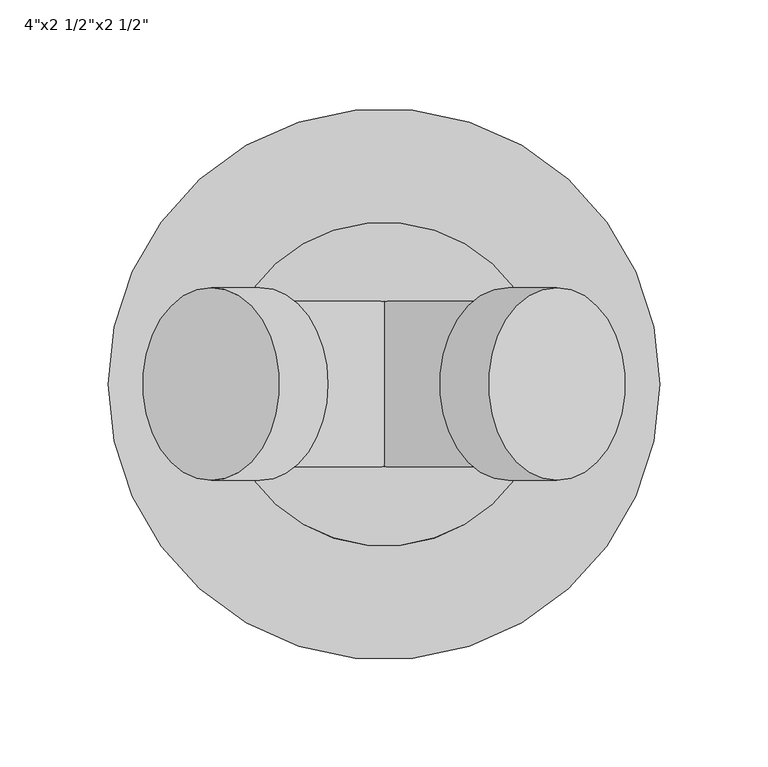
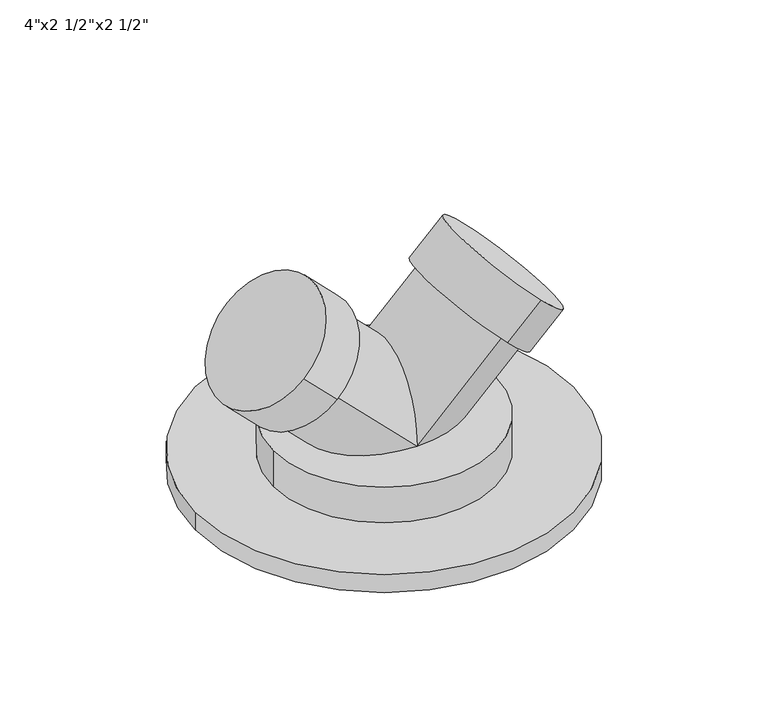
"""IFC4 building model written with IfcOpenShell, lengths in millimetres: proxy geometry."""

from ifc_helpers import new_model, si_unit, frame, origin, place, context, project, spatial, circle_curve, ellipse_curve, source, transform, mapped, element, save
from ifc_brep_helpers import plane_surface, cylinder_surface, advanced_brep


def proxy_83300ab8(model_context):
    return source(origin(), model_context, "Body", "AdvancedBrep", [
        advanced_brep(
        [(-127.0, 0.0, 0.0), (127.0, 0.0, 0.0), (-127.0, 0.0, 12.7), (127.0, 0.0, 12.7), (-74.6125, 0.0, 12.7), (74.6125, 0.0, 12.7), (-74.6125, 0.0, 38.1), (74.6125, 0.0, 38.1), (0.0, -38.1, 38.1), (0.0, 38.1, 38.1), (-57.2491328, 38.1, 95.3491328), (-57.2491328, -38.1, 95.3491328), (57.2491328, 38.1, 95.3491328), (57.2491328, -38.1, 95.3491328), (-57.2491328, 44.45, 95.3491328), (-57.2491328, -44.45, 95.3491328), (-79.6997731, 44.45, 117.7997731), (-79.6997731, -44.45, 117.7997731), (57.2491328, 44.45, 95.3491328), (57.2491328, -44.45, 95.3491328), (79.6997731, 44.45, 117.7997731), (79.6997731, -44.45, 117.7997731)],
        [
            (0, 1, circle_curve(frame((0.0, 0.0, 0.0), z_axis=(0.0, 0.0, -1.0), x_axis=(1.0, 0.0, 0.0)), 127.0)),
            (1, 0, circle_curve(frame((0.0, 0.0, 0.0), z_axis=(0.0, 0.0, -1.0), x_axis=(1.0, 0.0, 0.0)), 127.0)),
            (2, 3, circle_curve(frame((0.0, 0.0, 12.7), z_axis=(0.0, 0.0, 1.0), x_axis=(1.0, 0.0, 0.0)), 127.0)),
            (3, 2, circle_curve(frame((0.0, 0.0, 12.7), z_axis=(0.0, 0.0, 1.0), x_axis=(1.0, 0.0, 0.0)), 127.0)),
            (4, 5, circle_curve(frame((0.0, 0.0, 12.7), z_axis=(0.0, 0.0, -1.0), x_axis=(1.0, 0.0, 0.0)), 74.6125)),
            (5, 4, circle_curve(frame((0.0, 0.0, 12.7), z_axis=(0.0, 0.0, -1.0), x_axis=(1.0, 0.0, 0.0)), 74.6125)),
            (0, 2),
            (3, 1),
            (6, 7, circle_curve(frame((0.0, 0.0, 38.1), z_axis=(0.0, 0.0, 1.0), x_axis=(1.0, 0.0, 0.0)), 74.6125)),
            (7, 6, circle_curve(frame((0.0, 0.0, 38.1), z_axis=(0.0, 0.0, 1.0), x_axis=(1.0, 0.0, 0.0)), 74.6125)),
            (8, 9, ellipse_curve(frame((0.0, 0.0, 38.1), z_axis=(0.0, 0.0, -1.0), x_axis=(1.0, 0.0, 0.0)), 53.8815367, 38.1)),
            (9, 8, ellipse_curve(frame((0.0, 0.0, 38.1), z_axis=(0.0, 0.0, -1.0), x_axis=(-1.0, 0.0, 0.0)), 53.8815367, 38.1)),
            (7, 5),
            (4, 6),
            (9, 10),
            (10, 11, circle_curve(frame((-57.2491328, 0.0, 95.3491328), z_axis=(0.7071067811865458, 0.0, -0.7071067811865493), x_axis=(0.0, -1.0, 0.0)), 38.1)),
            (11, 8),
            (8, 9, ellipse_curve(frame((0.0, 0.0, 38.1), z_axis=(-1.0, 0.0, 0.0), x_axis=(0.0, 0.0, -1.0)), 53.8815367, 38.1)),
            (11, 10, circle_curve(frame((-57.2491328, 0.0, 95.3491328), z_axis=(0.7071067811865458, 0.0, -0.7071067811865493), x_axis=(0.0, -1.0, 0.0)), 38.1)),
            (9, 12),
            (12, 13, circle_curve(frame((57.2491328, 0.0, 95.3491328), z_axis=(-0.7071067811865603, 0.0, -0.7071067811865348), x_axis=(0.0, -1.0, 0.0)), 38.1)),
            (13, 8),
            (13, 12, circle_curve(frame((57.2491328, 0.0, 95.3491328), z_axis=(-0.7071067811865603, 0.0, -0.7071067811865348), x_axis=(0.0, -1.0, 0.0)), 38.1)),
            (14, 15, circle_curve(frame((-57.2491328, 0.0, 95.3491328), z_axis=(0.7071067811865429, 0.0, -0.7071067811865521), x_axis=(0.0, -1.0, 0.0)), 44.45)),
            (15, 14, circle_curve(frame((-57.2491328, 0.0, 95.3491328), z_axis=(0.7071067811865429, 0.0, -0.7071067811865521), x_axis=(0.0, -1.0, 0.0)), 44.45)),
            (16, 17, circle_curve(frame((-79.6997731, 0.0, 117.7997731), z_axis=(-0.7071067811865429, 0.0, 0.7071067811865521), x_axis=(0.0, -1.0, 0.0)), 44.45)),
            (17, 16, circle_curve(frame((-79.6997731, 0.0, 117.7997731), z_axis=(-0.7071067811865429, 0.0, 0.7071067811865521), x_axis=(0.0, -1.0, 0.0)), 44.45)),
            (14, 16),
            (17, 15),
            (18, 19, circle_curve(frame((57.2491328, 0.0, 95.3491328), z_axis=(-0.7071067811865575, 0.0, -0.7071067811865377), x_axis=(0.0, -1.0, 0.0)), 44.45)),
            (19, 18, circle_curve(frame((57.2491328, 0.0, 95.3491328), z_axis=(-0.7071067811865575, 0.0, -0.7071067811865377), x_axis=(0.0, -1.0, 0.0)), 44.45)),
            (20, 21, circle_curve(frame((79.6997731, 0.0, 117.7997731), z_axis=(0.7071067811865575, 0.0, 0.7071067811865377), x_axis=(0.0, -1.0, 0.0)), 44.45)),
            (21, 20, circle_curve(frame((79.6997731, 0.0, 117.7997731), z_axis=(0.7071067811865575, 0.0, 0.7071067811865377), x_axis=(0.0, -1.0, 0.0)), 44.45)),
            (18, 20),
            (21, 19),
        ],
        [
            plane_surface(frame((0.0, 0.0, 0.0), z_axis=(0.0, 0.0, -1.0), x_axis=(0.0, -1.0, 0.0))),
            plane_surface(frame((0.0, 0.0, 12.7), z_axis=(0.0, 0.0, 1.0), x_axis=(0.0, -1.0, 0.0))),
            cylinder_surface(frame((0.0, 0.0, 0.0), z_axis=(0.0, 0.0, -1.0), x_axis=(1.0, 0.0, 0.0)), 127.0),
            plane_surface(frame((0.0, 0.0, 38.1), z_axis=(0.0, 0.0, 1.0), x_axis=(0.0, -1.0, 0.0))),
            cylinder_surface(frame((0.0, 0.0, 12.7), z_axis=(0.0, 0.0, -1.0), x_axis=(1.0, 0.0, 0.0)), 74.6125),
            cylinder_surface(frame((0.0, 0.0, 38.1), z_axis=(0.7071067811865458, 0.0, -0.7071067811865493), x_axis=(0.0, -1.0, 0.0)), 38.1),
            cylinder_surface(frame((0.0, 0.0, 38.1), z_axis=(-0.7071067811865603, 0.0, -0.7071067811865348), x_axis=(0.0, -1.0, 0.0)), 38.1),
            plane_surface(frame((-57.2491328, 0.0, 95.3491328), z_axis=(0.707106781186543, 0.0, -0.7071067811865522), x_axis=(0.0, -1.0, 0.0))),
            plane_surface(frame((-79.6997731, 0.0, 117.7997731), z_axis=(-0.707106781186543, 0.0, 0.7071067811865522), x_axis=(0.0, -1.0, 0.0))),
            cylinder_surface(frame((-57.2491328, 0.0, 95.3491328), z_axis=(0.7071067811865429, 0.0, -0.7071067811865521), x_axis=(0.0, -1.0, 0.0)), 44.45),
            plane_surface(frame((57.2491328, 0.0, 95.3491328), z_axis=(-0.7071067811865575, 0.0, -0.7071067811865377), x_axis=(0.0, -1.0, 0.0))),
            plane_surface(frame((79.6997731, 0.0, 117.7997731), z_axis=(0.7071067811865575, 0.0, 0.7071067811865377), x_axis=(0.0, -1.0, 0.0))),
            cylinder_surface(frame((57.2491328, 0.0, 95.3491328), z_axis=(-0.7071067811865575, 0.0, -0.7071067811865377), x_axis=(0.0, -1.0, 0.0)), 44.45),
        ],
        [
            (0, [[1, 2]]),
            (1, [[3, 4], [5, 6]]),
            (2, [[-1, 7, -4, 8]]),
            (2, [[-2, -8, -3, -7]]),
            (3, [[9, 10], [11, 12]]),
            (4, [[-10, 13, -5, 14]]),
            (4, [[-9, -14, -6, -13]]),
            (5, [[15, 16, 17, 18]]),
            (5, [[-15, -11, -17, 19]]),
            (6, [[20, 21, 22, -12]]),
            (6, [[-20, -18, -22, 23]]),
            (7, [[24, 25], [-16, -19]]),
            (8, [[26, 27]]),
            (9, [[-24, 28, -27, 29]]),
            (9, [[-25, -29, -26, -28]]),
            (10, [[30, 31], [-21, -23]]),
            (11, [[32, 33]]),
            (12, [[-30, 34, -33, 35]]),
            (12, [[-31, -35, -32, -34]]),
        ],
    ),
    ])


if __name__ == "__main__":
    model = new_model("IFC4")
    model_context = context("Model", 3, world=origin())
    ifc_project = project(units=[si_unit("LENGTHUNIT", "METRE", prefix="MILLI")], contexts=[model_context])
    site = spatial("IfcSite", under=ifc_project)
    building = spatial("IfcBuilding", under=site)
    placement = place(None, origin())
    proxy_shape = proxy_83300ab8(model_context)
    element("IfcBuildingElementProxy", 1, Name="Fire Department Inlet Connection - 2 Way - Projecting : 4\"x2 1/2\"x2 1/2\"", ObjectType="Fire Department Inlet Connection - 2 Way - Projecting : 4\"x2 1/2\"x2 1/2\"", at=placement, inside=building, context=model_context, shape_type="MappedRepresentation", body=[
        mapped(proxy_shape, transform((0.0, 0.0, 0.0), x_axis=(1.0, 0.0, 0.0), y_axis=(0.0, 1.0, 0.0), z_axis=(0.0, 0.0, 1.0))),
    ])
    save(model, "model.ifc")

# Revit data of these elements
# Type "Fire Department Inlet Connection - 2 Way - Projecting : 4\"x2 1/2\"x2 1/2\""
#   Nominal Radius = 2"
#   Nominal Diameter = 4"
#   Default Elevation = 2' - 4"
#   Projecting Connection Material = none
